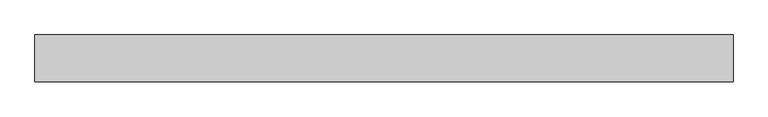
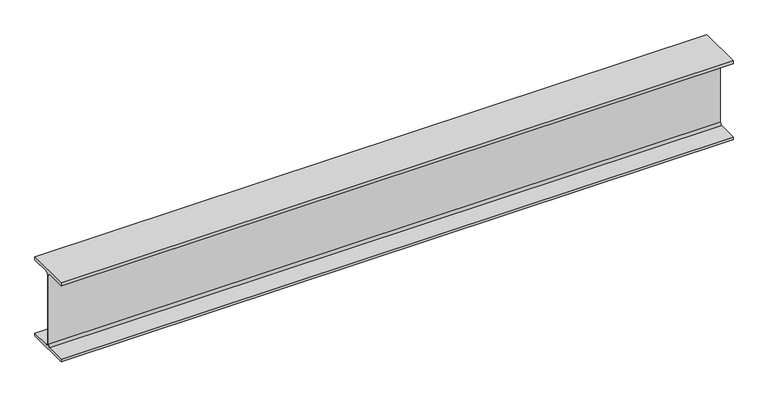
"""IFC4 building model written with IfcOpenShell, lengths in millimetres: beam geometry, Old_Steel Beam_H-KSD3502 : H_SB_ASB_H-194×150x6x9."""

import ifcopenshell
import ifcopenshell.guid

model = None  # the IFC model being written
_history = None  # IfcOwnerHistory: only IFC2X3 demands one
_inside = {}  # id of a spatial element -> (the spatial element, [elements in it])
_under = {}  # id of a project, library or spatial element -> (it, [spatial elements below it])
_declared = {}  # id of a project -> (the project, [libraries it declares])
_typed = {}  # id of a type object -> (the type object, [elements of that type])
_made_of = {}  # id of a material, layer set ... -> (it, [elements and type objects made of it])


def new_model(schema):
    """Start an empty IFC model of exactly this schema.

    Asked for "IFC4X3", IfcOpenShell would pick the latest addendum, in which some entities
    have other attributes; the version numbers below select the first issue.
    IFC2X3 requires an IfcOwnerHistory on every rooted entity: one is made here for all.
    """
    global model, _history
    if schema == "IFC4X3":
        model = ifcopenshell.file(schema_version=(4, 3, 0, 0))
    else:
        model = ifcopenshell.file(schema=schema)
    _inside.clear()
    _under.clear()
    _declared.clear()
    _typed.clear()
    _made_of.clear()
    _history = None
    if model.schema == "IFC2X3":
        org = make("IfcOrganization", Name="unknown")
        user = make(
            "IfcPersonAndOrganization",
            ThePerson=make("IfcPerson", FamilyName="unknown"),
            TheOrganization=org,
        )
        app = make(
            "IfcApplication",
            ApplicationDeveloper=org,
            Version="unknown",
            ApplicationFullName="unknown",
            ApplicationIdentifier="unknown",
        )
        _history = make(
            "IfcOwnerHistory",
            OwningUser=user,
            OwningApplication=app,
            ChangeAction="ADDED",
            CreationDate=0,
        )
    return model


def make(cls, **values):
    """One entity of the class cls with the attributes given. An attribute that is None is left unset."""
    return model.create_entity(
        cls, **{name: value for name, value in values.items() if value is not None}
    )


def rooted(cls, **values):
    """An entity with a GlobalId (a new one), such as an element, a storey or a relation."""
    return make(cls, GlobalId=ifcopenshell.guid.new(), OwnerHistory=_history, **values)


def si_unit(unit_type, name, prefix=None):
    """IfcSIUnit, for example si_unit("LENGTHUNIT", "METRE", prefix="MILLI")."""
    return make("IfcSIUnit", UnitType=unit_type, Prefix=prefix, Name=name)


def assignment(units):
    """IfcUnitAssignment: the units of a project."""
    return None if units is None else make("IfcUnitAssignment", Units=units)


def point(xyz):
    """IfcCartesianPoint."""
    return None if xyz is None else make("IfcCartesianPoint", Coordinates=xyz)


def direction(xyz):
    """IfcDirection."""
    return None if xyz is None else make("IfcDirection", DirectionRatios=xyz)


def frame(location, z_axis=None, x_axis=None):
    """IfcAxis2Placement3D, a coordinate frame: its origin and axes. An axis left out is left unset."""
    return make(
        "IfcAxis2Placement3D",
        Location=point(location),
        Axis=direction(z_axis),
        RefDirection=direction(x_axis),
    )


def frame_2d(location, x_axis=None):
    """IfcAxis2Placement2D, a coordinate frame in the plane: its origin and x axis."""
    return make(
        "IfcAxis2Placement2D", Location=point(location), RefDirection=direction(x_axis)
    )


def origin():
    """The frame at (0, 0, 0) with its axes left unset."""
    return frame((0.0, 0.0, 0.0))


def place(relative_to, where):
    """IfcLocalPlacement: puts the frame where relative to a parent placement (None: the world)."""
    return make(
        "IfcLocalPlacement", PlacementRelTo=relative_to, RelativePlacement=where
    )


def context(
    kind, dimensions, precision=None, world=None, true_north=None, identifier=None
):
    """IfcGeometricRepresentationContext, for example the 3D "Model" context."""
    return make(
        "IfcGeometricRepresentationContext",
        ContextIdentifier=identifier,
        ContextType=kind,
        CoordinateSpaceDimension=dimensions,
        Precision=precision,
        WorldCoordinateSystem=world,
        TrueNorth=true_north,
    )


def project(units=None, contexts=None):
    """IfcProject with its units and contexts."""
    return rooted(
        "IfcProject",
        Name="project",
        RepresentationContexts=contexts,
        UnitsInContext=assignment(units),
    )


def spatial(cls, under=None, at=None, **own):
    """A site, building, storey or space (cls), placed at a placement, below another one or the project."""
    s = rooted(cls, ObjectPlacement=at, **own)
    if under is not None:
        _under.setdefault(under.id(), (under, []))[1].append(s)
    return s


def polyline(points):
    """IfcPolyline through the points."""
    return make("IfcPolyline", Points=[point(p) for p in points])


def circle_curve(where, radius):
    """IfcCircle in the frame where."""
    return make("IfcCircle", Position=where, Radius=radius)


def trimmed(basis, trim1, trim2, sense, master):
    """IfcTrimmedCurve: the piece of a basis curve between two trims."""
    return make(
        "IfcTrimmedCurve",
        BasisCurve=basis,
        Trim1=trim1,
        Trim2=trim2,
        SenseAgreement=sense,
        MasterRepresentation=master,
    )


def segment(curve, same_sense, transition):
    """IfcCompositeCurveSegment."""
    return make(
        "IfcCompositeCurveSegment",
        Transition=transition,
        SameSense=same_sense,
        ParentCurve=curve,
    )


def composite_curve(segments, self_intersect=None):
    """IfcCompositeCurve: segments joined end to end."""
    return make("IfcCompositeCurve", Segments=segments, SelfIntersect=self_intersect)


def outline(outer, holes=None, kind="AREA"):
    """IfcArbitraryClosedProfileDef: a profile drawn as a closed curve; with holes, ...WithVoids."""
    if holes is None:
        return make("IfcArbitraryClosedProfileDef", ProfileType=kind, OuterCurve=outer)
    return make(
        "IfcArbitraryProfileDefWithVoids",
        ProfileType=kind,
        OuterCurve=outer,
        InnerCurves=holes,
    )


def extrude(swept, where, along, depth):
    """IfcExtrudedAreaSolid: the profile swept, set in the frame where, extruded along a direction by depth."""
    return make(
        "IfcExtrudedAreaSolid",
        SweptArea=swept,
        Position=where,
        ExtrudedDirection=direction(along),
        Depth=depth,
    )


def shape(context_of_items, identifier, shape_type, items):
    """IfcShapeRepresentation: the items that make up one representation, for example the "Body"."""
    return make(
        "IfcShapeRepresentation",
        ContextOfItems=context_of_items,
        RepresentationIdentifier=identifier,
        RepresentationType=shape_type,
        Items=items,
    )


def source(mapping_origin, context_of_items, identifier, shape_type, items):
    """IfcRepresentationMap: a shape defined once, which mapped items show again and again."""
    return make(
        "IfcRepresentationMap",
        MappingOrigin=mapping_origin,
        MappedRepresentation=shape(context_of_items, identifier, shape_type, items),
    )


def transform(
    local_origin,
    x_axis=None,
    y_axis=None,
    z_axis=None,
    scale=None,
    scale2=None,
    scale3=None,
    uniform=True,
):
    """IfcCartesianTransformationOperator3D, or its non-uniform kind. x_axis, y_axis, z_axis: its Axis1, 2, 3."""
    if uniform:
        return make(
            "IfcCartesianTransformationOperator3D",
            Axis1=direction(x_axis),
            Axis2=direction(y_axis),
            LocalOrigin=point(local_origin),
            Scale=scale,
            Axis3=direction(z_axis),
        )
    return make(
        "IfcCartesianTransformationOperator3DnonUniform",
        Axis1=direction(x_axis),
        Axis2=direction(y_axis),
        LocalOrigin=point(local_origin),
        Scale=scale,
        Axis3=direction(z_axis),
        Scale2=scale2,
        Scale3=scale3,
    )


def mapped(mapping_source, mapping_target):
    """IfcMappedItem: shows the shape of a source again, moved by a transform."""
    return make(
        "IfcMappedItem", MappingSource=mapping_source, MappingTarget=mapping_target
    )


def made_of(thing, what):
    """Note that an element or type object is made of a material, layer set ...; save() writes the relation."""
    if what is not None:
        _made_of.setdefault(what.id(), (what, []))[1].append(thing)
    return thing


def element(
    cls,
    number,
    at=None,
    inside=None,
    cuts=None,
    type_object=None,
    material=None,
    context=None,
    identifier="Body",
    shape_type=None,
    held_by="IfcProductDefinitionShape",
    body=None,
    shapes=None,
    **own,
):
    """One element of the class cls, such as IfcWall. Its Tag is "e" and its number.

    at: its placement. inside: the storey or other place that contains it. cuts: it is an
    opening in that element (IfcRelVoidsElement). A single representation is given by context,
    identifier, shape_type and body (its items); several are given by shapes. held_by: the class
    of the entity that holds the representations. save() writes the other relations.
    """
    e = rooted(cls, Tag="e%d" % number, ObjectPlacement=at, **own)
    if body is not None:
        shapes = [shape(context, identifier, shape_type, body)]
    if shapes is not None:
        e.Representation = make(held_by, Representations=shapes)
    if inside is not None:
        _inside.setdefault(inside.id(), (inside, []))[1].append(e)
    if cuts is not None:
        rooted(
            "IfcRelVoidsElement", RelatingBuildingElement=cuts, RelatedOpeningElement=e
        )
    if type_object is not None:
        _typed.setdefault(type_object.id(), (type_object, []))[1].append(e)
    return made_of(e, material)


def aggregate(whole, parts):
    """IfcRelAggregates: a whole, such as a stair, and the parts it consists of."""
    return rooted("IfcRelAggregates", RelatingObject=whole, RelatedObjects=parts)


def save(model, path):
    """Write the relations noted so far, then the file.

    IfcRelAggregates (storeys below a building ...), IfcRelContainedInSpatialStructure (elements
    in a storey), IfcRelDefinesByType, IfcRelAssociatesMaterial and IfcRelDeclares: one each for
    every whole, place, type object, material and project.
    """
    for whole, parts in _under.values():
        aggregate(whole, parts)
    for where, things in _inside.values():
        rooted(
            "IfcRelContainedInSpatialStructure",
            RelatedElements=things,
            RelatingStructure=where,
        )
    for kind, things in _typed.values():
        rooted("IfcRelDefinesByType", RelatedObjects=things, RelatingType=kind)
    for what, things in _made_of.values():
        rooted("IfcRelAssociatesMaterial", RelatedObjects=things, RelatingMaterial=what)
    for by, libraries in _declared.values():
        rooted("IfcRelDeclares", RelatingContext=by, RelatedDefinitions=libraries)
    model.write(path)


def beam_14fd6036(model_context):
    return source(origin(), model_context, "Body", "SweptSolid", [
        extrude(outline(composite_curve([segment(polyline([(-82.5, -141.5), (-11.9, -141.5)]), True, "CONTINUOUS"), segment(trimmed(circle_curve(frame_2d((-11.9, -132.6)), 8.9), [point((-11.9, -141.5))], [point((-3.0, -132.6))], True, "CARTESIAN"), True, "CONTINUOUS"), segment(polyline([(-3.0, -132.6), (-3.0, 132.6)]), True, "CONTINUOUS"), segment(trimmed(circle_curve(frame_2d((-11.9, 132.6)), 8.9), [point((-3.0, 132.6))], [point((-11.9, 141.5))], True, "CARTESIAN"), True, "CONTINUOUS"), segment(polyline([(-11.9, 141.5), (-82.5, 141.5), (-82.5, 151.7), (82.5, 151.7), (82.5, 141.5), (11.9, 141.5)]), True, "CONTINUOUS"), segment(trimmed(circle_curve(frame_2d((11.9, 132.6)), 8.9), [point((11.9, 141.5))], [point((3.0, 132.6))], True, "CARTESIAN"), True, "CONTINUOUS"), segment(polyline([(3.0, 132.6), (3.0, -132.6)]), True, "CONTINUOUS"), segment(trimmed(circle_curve(frame_2d((11.9, -132.6)), 8.9), [point((3.0, -132.6))], [point((11.9, -141.5))], True, "CARTESIAN"), True, "CONTINUOUS"), segment(polyline([(11.9, -141.5), (82.5, -141.5), (82.5, -151.7), (-82.5, -151.7), (-82.5, -141.5)]), True, "CONTINUOUS")], self_intersect=False)), frame((-1200.0, 0.0, 0.0), z_axis=(1.0, 0.0, 0.0), x_axis=(0.0, 1.0, 0.0)), (0.0, 0.0, 1.0), 2448.0465428),
    ])


if __name__ == "__main__":
    model = new_model("IFC4")
    model_context = context("Model", 3, world=origin())
    ifc_project = project(units=[si_unit("LENGTHUNIT", "METRE", prefix="MILLI")], contexts=[model_context])
    site = spatial("IfcSite", under=ifc_project)
    building = spatial("IfcBuilding", under=site)
    placement = place(None, origin())
    beam_shape = beam_14fd6036(model_context)
    element("IfcBeam", 1, ObjectType="Old_Steel Beam_H-KSD3502 : H_SB_ASB_H-194×150x6x9", at=placement, inside=building, context=model_context, shape_type="MappedRepresentation", body=[
        mapped(beam_shape, transform((0.0, 0.0, 0.0), x_axis=(1.0, 0.0, 0.0), y_axis=(0.0, 1.0, 0.0), z_axis=(0.0, 0.0, 1.0))),
    ])
    save(model, "model.ifc")

# Revit data of these elements
# Type "Old_Steel Beam_H-KSD3502 : H_SB_ASB_H-194×150x6x9"
#   Width = 15.0 cm
#   Web Thickness = 0.6 cm
#   Web Fillet = 1.3 cm
#   Warping Constant = 43316.0 cm⁶
#   Torsional Moment of Inertia = 8.622 cm⁴
#   Torsional Modulus = 1.0 cm³
#   Section Area = 39.01 cm²
#   Plastic Modulus weak axis = 104.0 cm³
#   Plastic Modulus strong axis = 309.0 cm³
#   Perimeter = 0.95 m²/m
#   Nominal Weight = 30.60 kgf/m
#   Moment of Inertia weak axis = 507.00 cm⁴
#   Moment of Inertia strong axis = 2690.00 cm⁴
#   Height = 19.4 cm
#   Flange Thickness = 0.9 cm
#   Elastic Modulus weak axis = 67.6 cm³
#   Elastic Modulus strong axis = 277.0 cm³
#   Centroid Vertical = 9.7 cm
#   Centroid Horizontal = 7.5 cm
#   Length [instance default] = 1.5240 m
#   Structural Material [instance default] = Steel, 45-345
#   Assembly Code = ""
# Element 1 (IfcBeam, "Old_Steel Beam_H-KSD3502 : H_SB_ASB_H-194×150x6x9")
#   Structural Material = none
# Materials
#   "Steel, 45-345": class "Metal", colour RGB 189 187 185, transparency 0, Description = "Steel 345 MPa", Cost = 0
